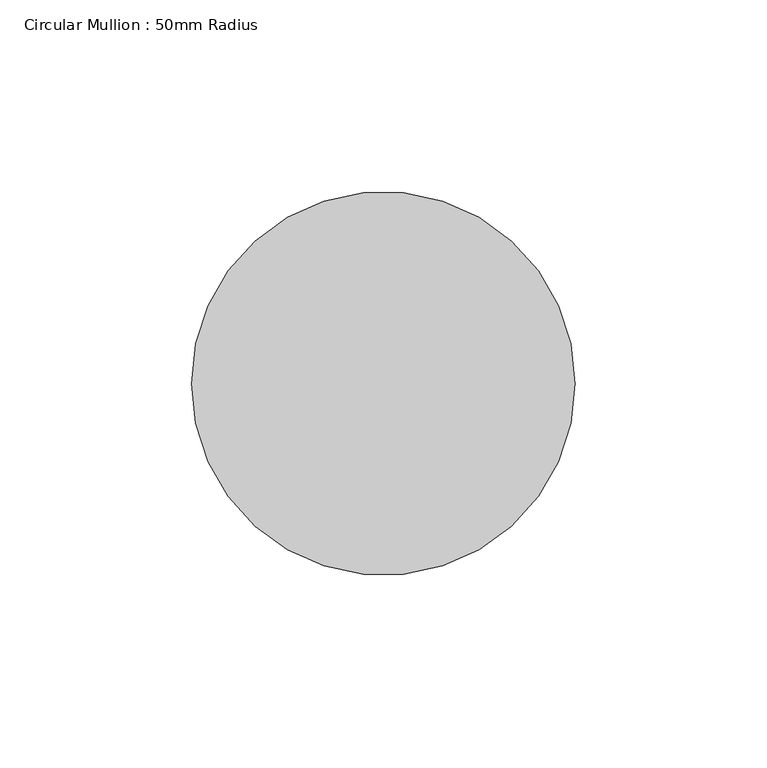
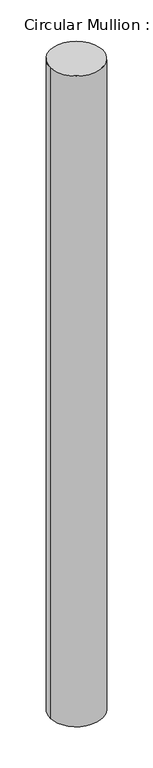
"""IFC4 building model written with IfcOpenShell, lengths in millimetres: member geometry, Circular Mullion : 50mm Radius."""

from ifc_helpers import new_model, si_unit, point, frame, origin, origin_2d, place, context, project, spatial, circle_curve, trimmed, segment, composite_curve, outline, extrude, source, transform, mapped, element, save


def circular_mullion_50mm_radius_0349539b(model_context):
    return source(origin(), model_context, "Body", "SweptSolid", [
        extrude(outline(composite_curve([segment(trimmed(circle_curve(origin_2d(), 50.0), [point((50.0, 0.0))], [point((-50.0, 0.0))], False, "CARTESIAN"), True, "CONTINUOUS"), segment(trimmed(circle_curve(origin_2d(), 50.0), [point((-50.0, 0.0))], [point((50.0, 0.0))], False, "CARTESIAN"), True, "CONTINUOUS")], self_intersect=False)), frame((0.0, 0.0, -1311.3299101), z_axis=(0.0, 0.0, 1.0), x_axis=(1.0, 0.0, 0.0)), (0.0, 0.0, 1.0), 1311.3299101),
    ])


if __name__ == "__main__":
    model = new_model("IFC4")
    model_context = context("Model", 3, world=origin())
    ifc_project = project(units=[si_unit("LENGTHUNIT", "METRE", prefix="MILLI")], contexts=[model_context])
    site = spatial("IfcSite", under=ifc_project)
    building = spatial("IfcBuilding", under=site)
    placement = place(None, origin())
    circular_mullion_50mm_radius_shape = circular_mullion_50mm_radius_0349539b(model_context)
    element("IfcMember", 1, ObjectType="Circular Mullion : 50mm Radius", at=placement, inside=building, context=model_context, shape_type="MappedRepresentation", body=[
        mapped(circular_mullion_50mm_radius_shape, transform((0.0, 0.0, 0.0), x_axis=(1.0, 0.0, 0.0), y_axis=(0.0, 1.0, 0.0), z_axis=(0.0, 0.0, 1.0))),
    ])
    save(model, "model.ifc")

# Revit data of these elements
# Type "Circular Mullion : 50mm Radius"
#   built-in parameter 1007350 = 0.164042 (stored number, unit not read)
# Element 1 (IfcMember, "Circular Mullion : 50mm Radius")
#   Materials on its faces: "Aluminium"
# Materials
#   "Aluminium": class "Metal", colour RGB 247 247 247, transparency 0, Description = "Aluminium 6061", Cost = 0
